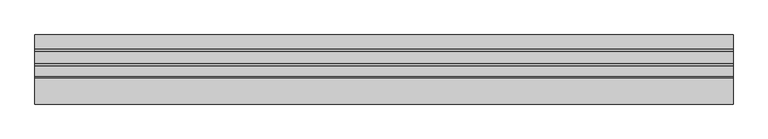
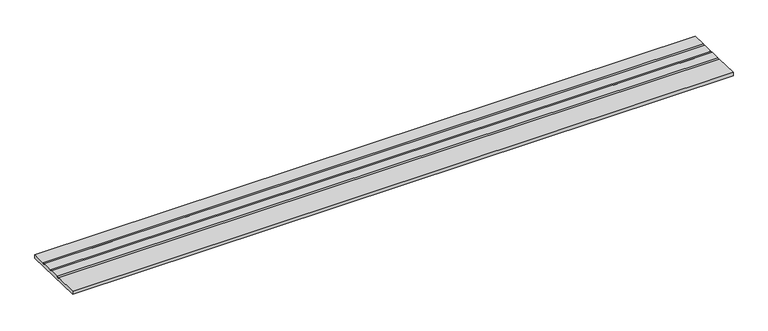
"""IFC4 building model written with IfcOpenShell, lengths in millimetres: proxy geometry, Generic Models 3:Generic Models 2:312240:Generic Models 2:312240 : Generic Models 3:Generic Models 2:312240:15 : Generic Models 3:Generic Models 2:312240:Generic Models 2:312240 : Generic Models 3:Generic Models 2:312240:300533."""

from ifc_helpers import new_model, si_unit, point, frame, frame_2d, origin, place, context, project, spatial, polyline, circle_curve, trimmed, segment, composite_curve, outline, extrude, source, transform, mapped, element, save


def generic_models_17313230(model_context):
    return source(origin(), model_context, "Body", "SweptSolid", [
        extrude(outline(composite_curve([segment(polyline([(-579013.3913841, 1320.5988067), (-579013.3913841, 1333.3015625), (-578924.0467323, 1331.4402156)]), True, "CONTINUOUS"), segment(trimmed(circle_curve(frame_2d((-578919.8539034, 1332.9784188)), 4.4660814), [point((-578924.0467323, 1331.4402156))], [point((-578915.7287766, 1331.2669248))], True, "CARTESIAN"), True, "CONTINUOUS"), segment(polyline([(-578915.7287766, 1331.2669248), (-578879.1424508, 1330.5047097)]), True, "CONTINUOUS"), segment(trimmed(circle_curve(frame_2d((-578874.9942916, 1332.1595987)), 4.4660814), [point((-578879.1424508, 1330.5047097))], [point((-578870.9186554, 1330.3333807))], True, "CARTESIAN"), True, "CONTINUOUS"), segment(polyline([(-578870.9186554, 1330.3333807), (-578830.9091735, 1329.4998498)]), True, "CONTINUOUS"), segment(trimmed(circle_curve(frame_2d((-578826.7610142, 1331.1547388)), 4.4660814), [point((-578830.9091735, 1329.4998498))], [point((-578822.685378, 1329.3285207))], True, "CARTESIAN"), True, "CONTINUOUS"), segment(polyline([(-578822.685378, 1329.3285207), (-578771.8963988, 1328.270417), (-578772.1609247, 1315.5731722), (-579013.3913841, 1320.5988067)]), True, "CONTINUOUS")], self_intersect=False)), frame((590317.0242239, 0.0, 0.0), z_axis=(1.0, 0.0, 0.0), x_axis=(0.0, 1.0, 0.0)), (0.0, 0.0, 1.0), 2438.4),
    ])


if __name__ == "__main__":
    model = new_model("IFC4")
    model_context = context("Model", 3, world=origin())
    ifc_project = project(units=[si_unit("LENGTHUNIT", "METRE", prefix="MILLI")], contexts=[model_context])
    site = spatial("IfcSite", under=ifc_project)
    building = spatial("IfcBuilding", under=site)
    placement = place(None, origin())
    generic_models_shape = generic_models_17313230(model_context)
    element("IfcBuildingElementProxy", 1, Name="Generic Models 3:Generic Models 2:312240:Generic Models 2:312240 : Generic Models 3:Generic Models 2:312240:15 : Generic Models 3:Generic Models 2:312240:Generic Models 2:312240 : Generic Models 3:Generic Models 2:312240:300533", ObjectType="Generic Models 3:Generic Models 2:312240:Generic Models 2:312240 : Generic Models 3:Generic Models 2:312240:15 : Generic Models 3:Generic Models 2:312240:Generic Models 2:312240 : Generic Models 3:Generic Models 2:312240:300533", at=placement, inside=building, context=model_context, shape_type="MappedRepresentation", body=[
        mapped(generic_models_shape, transform((0.0, 0.0, 0.0), x_axis=(1.0, 0.0, 0.0), y_axis=(0.0, 1.0, 0.0), z_axis=(0.0, 0.0, 1.0))),
    ])
    save(model, "model.ifc")

# Revit data of these elements
# Type "Generic Models 3:Generic Models 2:312240:Generic Models 2:312240 : Generic Models 3:Generic Models 2:312240:15 : Generic Models 3:Generic Models 2:312240:Generic Models 2:312240 : Generic Models 3:Generic Models 2:312240:300533"
#   NameOverride = "Generic Models 3:Generic Models 2:312240:Generic Models 2:312240 : Generic Models 3:Generic Models 2:312240:300533"
#   ObjectTypeOverride = "Generic Models 2:312240 : Generic Models 3:Generic Models 2:312240"
#   Reference = "Generic Models 2"
#   Tag = "300533"
# Element 1 (IfcBuildingElementProxy, "Generic Models 3:Generic Models 2:312240:Generic Models 2:312240 : Generic Models 3:Generic Models 2:312240:15 : Generic Models 3:Generic Models 2:312240:Generic Models 2:312240 : Generic Models 3:Generic Models 2:312240:300533")
#   Materials on its faces: "SOLID SURFACE MATERIAL (WITH HARD SEAMS, UNLESS OTHERWISE NOTED)"
# Materials
#   "SOLID SURFACE MATERIAL (WITH HARD SEAMS, UNLESS OTHERWISE NOTED)": class "Generic", colour RGB 242 242 242, transparency 0, Cost = 0
